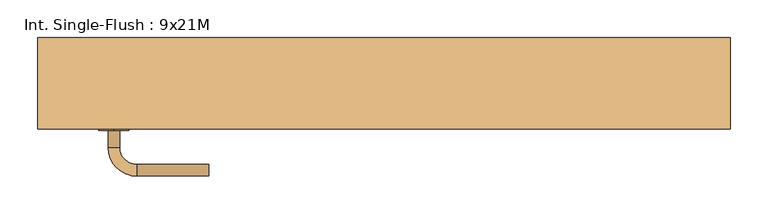
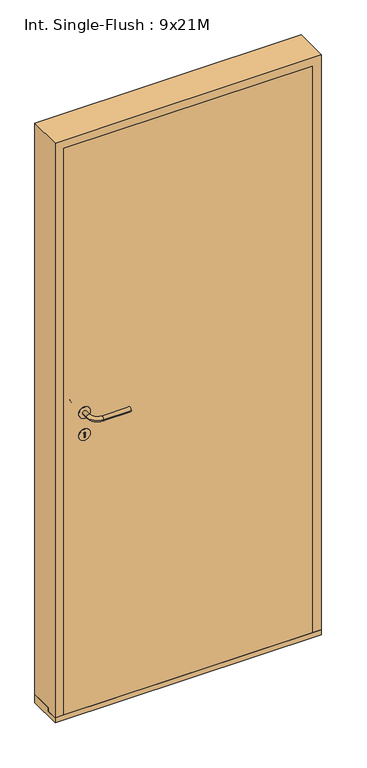
"""IFC4 building model written with IfcOpenShell, lengths in millimetres: door geometry, Int. Single-Flush : 9x21M."""

import ifcopenshell
import ifcopenshell.guid

model = None  # the IFC model being written
_history = None  # IfcOwnerHistory: only IFC2X3 demands one
_inside = {}  # id of a spatial element -> (the spatial element, [elements in it])
_under = {}  # id of a project, library or spatial element -> (it, [spatial elements below it])
_declared = {}  # id of a project -> (the project, [libraries it declares])
_typed = {}  # id of a type object -> (the type object, [elements of that type])
_made_of = {}  # id of a material, layer set ... -> (it, [elements and type objects made of it])


def new_model(schema):
    """Start an empty IFC model of exactly this schema.

    Asked for "IFC4X3", IfcOpenShell would pick the latest addendum, in which some entities
    have other attributes; the version numbers below select the first issue.
    IFC2X3 requires an IfcOwnerHistory on every rooted entity: one is made here for all.
    """
    global model, _history
    if schema == "IFC4X3":
        model = ifcopenshell.file(schema_version=(4, 3, 0, 0))
    else:
        model = ifcopenshell.file(schema=schema)
    _inside.clear()
    _under.clear()
    _declared.clear()
    _typed.clear()
    _made_of.clear()
    _history = None
    if model.schema == "IFC2X3":
        org = make("IfcOrganization", Name="unknown")
        user = make(
            "IfcPersonAndOrganization",
            ThePerson=make("IfcPerson", FamilyName="unknown"),
            TheOrganization=org,
        )
        app = make(
            "IfcApplication",
            ApplicationDeveloper=org,
            Version="unknown",
            ApplicationFullName="unknown",
            ApplicationIdentifier="unknown",
        )
        _history = make(
            "IfcOwnerHistory",
            OwningUser=user,
            OwningApplication=app,
            ChangeAction="ADDED",
            CreationDate=0,
        )
    return model


def make(cls, **values):
    """One entity of the class cls with the attributes given. An attribute that is None is left unset."""
    return model.create_entity(
        cls, **{name: value for name, value in values.items() if value is not None}
    )


def rooted(cls, **values):
    """An entity with a GlobalId (a new one), such as an element, a storey or a relation."""
    return make(cls, GlobalId=ifcopenshell.guid.new(), OwnerHistory=_history, **values)


def si_unit(unit_type, name, prefix=None):
    """IfcSIUnit, for example si_unit("LENGTHUNIT", "METRE", prefix="MILLI")."""
    return make("IfcSIUnit", UnitType=unit_type, Prefix=prefix, Name=name)


def assignment(units):
    """IfcUnitAssignment: the units of a project."""
    return None if units is None else make("IfcUnitAssignment", Units=units)


def point(xyz):
    """IfcCartesianPoint."""
    return None if xyz is None else make("IfcCartesianPoint", Coordinates=xyz)


def direction(xyz):
    """IfcDirection."""
    return None if xyz is None else make("IfcDirection", DirectionRatios=xyz)


def frame(location, z_axis=None, x_axis=None):
    """IfcAxis2Placement3D, a coordinate frame: its origin and axes. An axis left out is left unset."""
    return make(
        "IfcAxis2Placement3D",
        Location=point(location),
        Axis=direction(z_axis),
        RefDirection=direction(x_axis),
    )


def frame_2d(location, x_axis=None):
    """IfcAxis2Placement2D, a coordinate frame in the plane: its origin and x axis."""
    return make(
        "IfcAxis2Placement2D", Location=point(location), RefDirection=direction(x_axis)
    )


def origin():
    """The frame at (0, 0, 0) with its axes left unset."""
    return frame((0.0, 0.0, 0.0))


def place(relative_to, where):
    """IfcLocalPlacement: puts the frame where relative to a parent placement (None: the world)."""
    return make(
        "IfcLocalPlacement", PlacementRelTo=relative_to, RelativePlacement=where
    )


def context(
    kind, dimensions, precision=None, world=None, true_north=None, identifier=None
):
    """IfcGeometricRepresentationContext, for example the 3D "Model" context."""
    return make(
        "IfcGeometricRepresentationContext",
        ContextIdentifier=identifier,
        ContextType=kind,
        CoordinateSpaceDimension=dimensions,
        Precision=precision,
        WorldCoordinateSystem=world,
        TrueNorth=true_north,
    )


def project(units=None, contexts=None):
    """IfcProject with its units and contexts."""
    return rooted(
        "IfcProject",
        Name="project",
        RepresentationContexts=contexts,
        UnitsInContext=assignment(units),
    )


def spatial(cls, under=None, at=None, **own):
    """A site, building, storey or space (cls), placed at a placement, below another one or the project."""
    s = rooted(cls, ObjectPlacement=at, **own)
    if under is not None:
        _under.setdefault(under.id(), (under, []))[1].append(s)
    return s


def polyline(points):
    """IfcPolyline through the points."""
    return make("IfcPolyline", Points=[point(p) for p in points])


def circle_curve(where, radius):
    """IfcCircle in the frame where."""
    return make("IfcCircle", Position=where, Radius=radius)


def ellipse_curve(where, semi_axis1, semi_axis2):
    """IfcEllipse in the frame where."""
    return make(
        "IfcEllipse", Position=where, SemiAxis1=semi_axis1, SemiAxis2=semi_axis2
    )


def trimmed(basis, trim1, trim2, sense, master):
    """IfcTrimmedCurve: the piece of a basis curve between two trims."""
    return make(
        "IfcTrimmedCurve",
        BasisCurve=basis,
        Trim1=trim1,
        Trim2=trim2,
        SenseAgreement=sense,
        MasterRepresentation=master,
    )


def segment(curve, same_sense, transition):
    """IfcCompositeCurveSegment."""
    return make(
        "IfcCompositeCurveSegment",
        Transition=transition,
        SameSense=same_sense,
        ParentCurve=curve,
    )


def composite_curve(segments, self_intersect=None):
    """IfcCompositeCurve: segments joined end to end."""
    return make("IfcCompositeCurve", Segments=segments, SelfIntersect=self_intersect)


def outline(outer, holes=None, kind="AREA"):
    """IfcArbitraryClosedProfileDef: a profile drawn as a closed curve; with holes, ...WithVoids."""
    if holes is None:
        return make("IfcArbitraryClosedProfileDef", ProfileType=kind, OuterCurve=outer)
    return make(
        "IfcArbitraryProfileDefWithVoids",
        ProfileType=kind,
        OuterCurve=outer,
        InnerCurves=holes,
    )


def extrude(swept, where, along, depth):
    """IfcExtrudedAreaSolid: the profile swept, set in the frame where, extruded along a direction by depth."""
    return make(
        "IfcExtrudedAreaSolid",
        SweptArea=swept,
        Position=where,
        ExtrudedDirection=direction(along),
        Depth=depth,
    )


def faces_of(points, faces, orient=None, outer=None):
    """IfcFace entities. A face is a list of loops; a loop is a list of indices into points, from 0.

    orient and outer hold one flag for each loop. By default every Orientation is true, the
    first loop of a face is its IfcFaceOuterBound and the others are IfcFaceBound.
    """
    made = []
    for i, loops in enumerate(faces):
        bounds = []
        for j, loop in enumerate(loops):
            is_outer = j == 0 if outer is None else outer[i][j]
            bounds.append(
                make(
                    "IfcFaceOuterBound" if is_outer else "IfcFaceBound",
                    Bound=make("IfcPolyLoop", Polygon=[points[k] for k in loop]),
                    Orientation=True if orient is None else orient[i][j],
                )
            )
        made.append(make("IfcFace", Bounds=bounds))
    return made


def faceted_brep(points, faces, orient=None, outer=None, voids=None):
    """IfcFacetedBrep: a solid bounded by flat faces; with voids (closed shells), ...WithVoids."""
    shared = [point(p) for p in points]
    hull = make("IfcClosedShell", CfsFaces=faces_of(shared, faces, orient, outer))
    if voids is None:
        return make("IfcFacetedBrep", Outer=hull)
    return make(
        "IfcFacetedBrepWithVoids",
        Outer=hull,
        Voids=[
            make(cls, CfsFaces=faces_of(shared, fs, o, b)) for cls, fs, o, b in voids
        ],
    )


def shape(context_of_items, identifier, shape_type, items):
    """IfcShapeRepresentation: the items that make up one representation, for example the "Body"."""
    return make(
        "IfcShapeRepresentation",
        ContextOfItems=context_of_items,
        RepresentationIdentifier=identifier,
        RepresentationType=shape_type,
        Items=items,
    )


def source(mapping_origin, context_of_items, identifier, shape_type, items):
    """IfcRepresentationMap: a shape defined once, which mapped items show again and again."""
    return make(
        "IfcRepresentationMap",
        MappingOrigin=mapping_origin,
        MappedRepresentation=shape(context_of_items, identifier, shape_type, items),
    )


def transform(
    local_origin,
    x_axis=None,
    y_axis=None,
    z_axis=None,
    scale=None,
    scale2=None,
    scale3=None,
    uniform=True,
):
    """IfcCartesianTransformationOperator3D, or its non-uniform kind. x_axis, y_axis, z_axis: its Axis1, 2, 3."""
    if uniform:
        return make(
            "IfcCartesianTransformationOperator3D",
            Axis1=direction(x_axis),
            Axis2=direction(y_axis),
            LocalOrigin=point(local_origin),
            Scale=scale,
            Axis3=direction(z_axis),
        )
    return make(
        "IfcCartesianTransformationOperator3DnonUniform",
        Axis1=direction(x_axis),
        Axis2=direction(y_axis),
        LocalOrigin=point(local_origin),
        Scale=scale,
        Axis3=direction(z_axis),
        Scale2=scale2,
        Scale3=scale3,
    )


def mapped(mapping_source, mapping_target):
    """IfcMappedItem: shows the shape of a source again, moved by a transform."""
    return make(
        "IfcMappedItem", MappingSource=mapping_source, MappingTarget=mapping_target
    )


def made_of(thing, what):
    """Note that an element or type object is made of a material, layer set ...; save() writes the relation."""
    if what is not None:
        _made_of.setdefault(what.id(), (what, []))[1].append(thing)
    return thing


def element(
    cls,
    number,
    at=None,
    inside=None,
    cuts=None,
    type_object=None,
    material=None,
    context=None,
    identifier="Body",
    shape_type=None,
    held_by="IfcProductDefinitionShape",
    body=None,
    shapes=None,
    **own,
):
    """One element of the class cls, such as IfcWall. Its Tag is "e" and its number.

    at: its placement. inside: the storey or other place that contains it. cuts: it is an
    opening in that element (IfcRelVoidsElement). A single representation is given by context,
    identifier, shape_type and body (its items); several are given by shapes. held_by: the class
    of the entity that holds the representations. save() writes the other relations.
    """
    e = rooted(cls, Tag="e%d" % number, ObjectPlacement=at, **own)
    if body is not None:
        shapes = [shape(context, identifier, shape_type, body)]
    if shapes is not None:
        e.Representation = make(held_by, Representations=shapes)
    if inside is not None:
        _inside.setdefault(inside.id(), (inside, []))[1].append(e)
    if cuts is not None:
        rooted(
            "IfcRelVoidsElement", RelatingBuildingElement=cuts, RelatedOpeningElement=e
        )
    if type_object is not None:
        _typed.setdefault(type_object.id(), (type_object, []))[1].append(e)
    return made_of(e, material)


def aggregate(whole, parts):
    """IfcRelAggregates: a whole, such as a stair, and the parts it consists of."""
    return rooted("IfcRelAggregates", RelatingObject=whole, RelatedObjects=parts)


def save(model, path):
    """Write the relations noted so far, then the file.

    IfcRelAggregates (storeys below a building ...), IfcRelContainedInSpatialStructure (elements
    in a storey), IfcRelDefinesByType, IfcRelAssociatesMaterial and IfcRelDeclares: one each for
    every whole, place, type object, material and project.
    """
    for whole, parts in _under.values():
        aggregate(whole, parts)
    for where, things in _inside.values():
        rooted(
            "IfcRelContainedInSpatialStructure",
            RelatedElements=things,
            RelatingStructure=where,
        )
    for kind, things in _typed.values():
        rooted("IfcRelDefinesByType", RelatedObjects=things, RelatingType=kind)
    for what, things in _made_of.values():
        rooted("IfcRelAssociatesMaterial", RelatedObjects=things, RelatingMaterial=what)
    for by, libraries in _declared.values():
        rooted("IfcRelDeclares", RelatingContext=by, RelatedDefinitions=libraries)
    model.write(path)


def plane_surface(at):
    """IfcPlane: the flat surface through the origin of the frame at, square to its z axis."""
    return make("IfcPlane", Position=at)


def cylinder_surface(at, radius):
    """IfcCylindricalSurface: all points at the distance radius from the z axis of the frame at."""
    return make("IfcCylindricalSurface", Position=at, Radius=radius)


def revolved_surface(curve, axis_point, axis_direction):
    """IfcSurfaceOfRevolution: the curve turned about the line through axis_point along axis_direction."""
    return make(
        "IfcSurfaceOfRevolution",
        SweptCurve=make("IfcArbitraryOpenProfileDef", ProfileType="CURVE", Curve=curve),
        AxisPosition=make("IfcAxis1Placement", Location=point(axis_point), Axis=direction(axis_direction)),
    )


def advanced_brep(points, edges, surfaces, faces):
    """IfcAdvancedBrep: a solid bounded by faces that lie on surfaces and meet in shared edges.

    An edge is (start, end): straight between two places in points (the first is 0);
    or (start, end, curve); or (start, end, curve, False) where it runs against its curve.
    A face is (place in surfaces, loops), or (place, loops, False) where it looks against
    its surface's normal. A loop lists edges by number (the first is 1), with a minus sign
    where the edge is run from its end to its start. The first loop is the outer one.
    """
    corners = [point(p) for p in points]
    vertices = [make("IfcVertexPoint", VertexGeometry=c) for c in corners]
    made = []
    for start, end, *more in edges:
        made.append(
            make(
                "IfcEdgeCurve",
                EdgeStart=vertices[start],
                EdgeEnd=vertices[end],
                EdgeGeometry=more[0] if more else make("IfcPolyline", Points=[corners[start], corners[end]]),
                SameSense=more[1] if len(more) > 1 else True,
            )
        )
    hull = []
    for where, loops, *sense in faces:
        bounds = []
        for j, loop in enumerate(loops):
            ring = [make("IfcOrientedEdge", EdgeElement=made[abs(k) - 1], Orientation=k > 0) for k in loop]
            bounds.append(
                make(
                    "IfcFaceOuterBound" if j == 0 else "IfcFaceBound",
                    Bound=make("IfcEdgeLoop", EdgeList=ring),
                    Orientation=True,
                )
            )
        hull.append(make("IfcAdvancedFace", Bounds=bounds, FaceSurface=surfaces[where], SameSense=sense[0] if sense else True))
    return make("IfcAdvancedBrep", Outer=make("IfcClosedShell", CfsFaces=hull))


def int_single_flush_9x21m_9bb4a9f8(model_context):
    return source(origin(), model_context, "Body", "SolidModel", [
        extrude(outline(composite_curve([segment(trimmed(circle_curve(frame_2d((1090.0, -356.0)), 20.0), [point((1070.0, -356.0))], [point((1110.0, -356.0))], False, "CARTESIAN"), True, "CONTINUOUS"), segment(trimmed(circle_curve(frame_2d((1090.0, -356.0)), 20.0), [point((1110.0, -356.0))], [point((1070.0, -356.0))], False, "CARTESIAN"), True, "CONTINUOUS")], self_intersect=False)), frame((0.0, -62.0, 0.0), z_axis=(0.0, 1.0, 0.0), x_axis=(0.0, 0.0, 1.0)), (0.0, 0.0, 1.0), 2.0),
        advanced_brep(
        [(-363.5, -62.0, 1090.0), (-348.5, -62.0, 1090.0), (-348.5, -84.5, 1090.0), (-363.5, -84.5, 1090.0), (-326.0, -107.0, 1090.0), (-326.0, -122.0, 1090.0), (-231.0, -107.0, 1090.0), (-231.0, -122.0, 1090.0)],
        [
            (0, 1, circle_curve(frame((-356.0, -62.0, 1090.0), z_axis=(0.0, 1.0, 0.0), x_axis=(1.0, 0.0, 0.0)), 7.5)),
            (1, 0, circle_curve(frame((-356.0, -62.0, 1090.0), z_axis=(0.0, 1.0, 0.0), x_axis=(1.0, 0.0, 0.0)), 7.5)),
            (1, 2),
            (2, 3, circle_curve(frame((-356.0, -84.5, 1090.0), z_axis=(0.0, 1.0, 0.0), x_axis=(1.0, 0.0, 0.0)), 7.5)),
            (3, 0),
            (3, 2, circle_curve(frame((-356.0, -84.5, 1090.0), z_axis=(0.0, 1.0, 0.0), x_axis=(1.0, 0.0, 0.0)), 7.5)),
            (4, 5, circle_curve(frame((-326.0, -114.5, 1090.0), z_axis=(-1.0, 0.0, 0.0), x_axis=(0.0, 1.0, 0.0)), 7.5)),
            (5, 3, circle_curve(frame((-326.0, -84.5, 1090.0), z_axis=(0.0, 0.0, -1.0), x_axis=(-1.0, 0.0, 0.0)), 37.5)),
            (2, 4, circle_curve(frame((-326.0, -84.5, 1090.0), z_axis=(0.0, 0.0, 1.0), x_axis=(-1.0, 0.0, 0.0)), 22.5)),
            (5, 4, circle_curve(frame((-326.0, -114.5, 1090.0), z_axis=(-1.0, 0.0, 0.0), x_axis=(0.0, 1.0, 0.0)), 7.5)),
            (4, 6),
            (6, 7, circle_curve(frame((-231.0, -114.5, 1090.0), z_axis=(-1.0, 0.0, 0.0), x_axis=(0.0, 1.0, 0.0)), 7.5)),
            (7, 5),
            (7, 6, circle_curve(frame((-231.0, -114.5, 1090.0), z_axis=(-1.0, 0.0, 0.0), x_axis=(0.0, 1.0, 0.0)), 7.5)),
        ],
        [
            plane_surface(frame((-356.0, -62.0, 1090.0), z_axis=(0.0, 1.0, 0.0), x_axis=(0.0, 0.0, -1.0))),
            cylinder_surface(frame((-356.0, -62.0, 1090.0), z_axis=(0.0, 1.0, 0.0), x_axis=(1.0, 0.0, 0.0)), 7.5),
            revolved_surface(trimmed(ellipse_curve(frame((-356.0, -84.5, 1090.0), z_axis=(0.0, -1.0, 0.0), x_axis=(1.0, 0.0, 0.0)), 7.5, 7.5), [point((-363.5, -84.5, 1090.0))], [point((-348.5, -84.5, 1090.0))], True, "CARTESIAN"), (-326.0, -84.5, 1090.0), (0.0, 0.0, -1.0)),
            revolved_surface(trimmed(ellipse_curve(frame((-356.0, -84.5, 1090.0), z_axis=(0.0, -1.0, 0.0), x_axis=(1.0, 0.0, 0.0)), 7.5, 7.5), [point((-348.5, -84.5, 1090.0))], [point((-363.5, -84.5, 1090.0))], True, "CARTESIAN"), (-326.0, -84.5, 1090.0), (0.0, 0.0, -1.0)),
            cylinder_surface(frame((-326.0, -114.5, 1090.0), z_axis=(-1.0, 0.0, 0.0), x_axis=(0.0, 1.0, 0.0)), 7.5),
            plane_surface(frame((-231.0, -114.5, 1090.0), z_axis=(1.0, 0.0, 0.0), x_axis=(0.0, 0.0, -1.0))),
        ],
        [
            (0, [[1, 2]]),
            (1, [[3, 4, 5, -2]]),
            (1, [[-5, 6, -3, -1]]),
            (2, [[7, 8, -4, 9]]),
            (3, [[10, -9, -6, -8]]),
            (4, [[11, 12, 13, -7]]),
            (4, [[-13, 14, -11, -10]]),
            (5, [[-12, -14]]),
        ],
    ),
        extrude(outline(composite_curve([segment(trimmed(circle_curve(frame_2d((1010.0, -356.0)), 20.0), [point((990.0, -356.0))], [point((1030.0, -356.0))], False, "CARTESIAN"), True, "CONTINUOUS"), segment(trimmed(circle_curve(frame_2d((1010.0, -356.0)), 20.0), [point((1030.0, -356.0))], [point((990.0, -356.0))], False, "CARTESIAN"), True, "CONTINUOUS")], self_intersect=False), holes=[composite_curve([segment(trimmed(circle_curve(frame_2d((1015.0, -356.0)), 3.0), [point((1012.4019238, -357.5))], [point((1012.4019238, -354.5))], True, "CARTESIAN"), True, "CONTINUOUS"), segment(polyline([(1012.4019238, -354.5), (1000.0, -354.5), (1000.0, -357.5), (1012.4019238, -357.5)]), True, "CONTINUOUS")], self_intersect=False)]), frame((0.0, -62.0, 0.0), z_axis=(0.0, 1.0, 0.0), x_axis=(0.0, 0.0, 1.0)), (0.0, 0.0, 1.0), 2.0),
        extrude(outline(composite_curve([segment(trimmed(circle_curve(frame_2d((1090.0, -356.0)), 20.0), [point((1070.0, -356.0))], [point((1110.0, -356.0))], False, "CARTESIAN"), True, "CONTINUOUS"), segment(trimmed(circle_curve(frame_2d((1090.0, -356.0)), 20.0), [point((1110.0, -356.0))], [point((1070.0, -356.0))], False, "CARTESIAN"), True, "CONTINUOUS")], self_intersect=False)), frame((0.0, -20.0, 0.0), z_axis=(0.0, 1.0, 0.0), x_axis=(0.0, 0.0, 1.0)), (0.0, 0.0, 1.0), 2.0),
        advanced_brep(
        [(-363.5, -18.0, 1090.0), (-348.5, -18.0, 1090.0), (-363.5, 4.5, 1090.0), (-348.5, 4.5, 1090.0), (-326.0, 27.0, 1090.0), (-326.0, 42.0, 1090.0), (-231.0, 42.0, 1090.0), (-231.0, 27.0, 1090.0)],
        [
            (0, 1, circle_curve(frame((-356.0, -18.0, 1090.0), z_axis=(0.0, -1.0, 0.0), x_axis=(1.0, 0.0, 0.0)), 7.5)),
            (1, 0, circle_curve(frame((-356.0, -18.0, 1090.0), z_axis=(0.0, -1.0, 0.0), x_axis=(1.0, 0.0, 0.0)), 7.5)),
            (0, 2),
            (2, 3, circle_curve(frame((-356.0, 4.5, 1090.0), z_axis=(0.0, -1.0, 0.0), x_axis=(1.0, 0.0, 0.0)), 7.5)),
            (3, 1),
            (3, 2, circle_curve(frame((-356.0, 4.5, 1090.0), z_axis=(0.0, -1.0, 0.0), x_axis=(1.0, 0.0, 0.0)), 7.5)),
            (4, 3, circle_curve(frame((-326.0, 4.5, 1090.0), z_axis=(0.0, 0.0, 1.0), x_axis=(-1.0, 0.0, 0.0)), 22.5)),
            (2, 5, circle_curve(frame((-326.0, 4.5, 1090.0), z_axis=(0.0, 0.0, -1.0), x_axis=(-1.0, 0.0, 0.0)), 37.5)),
            (5, 4, circle_curve(frame((-326.0, 34.5, 1090.0), z_axis=(-1.0, 0.0, 0.0), x_axis=(0.0, -1.0, 0.0)), 7.5)),
            (4, 5, circle_curve(frame((-326.0, 34.5, 1090.0), z_axis=(-1.0, 0.0, 0.0), x_axis=(0.0, -1.0, 0.0)), 7.5)),
            (5, 6),
            (6, 7, circle_curve(frame((-231.0, 34.5, 1090.0), z_axis=(-1.0, 0.0, 0.0), x_axis=(0.0, -1.0, 0.0)), 7.5)),
            (7, 4),
            (7, 6, circle_curve(frame((-231.0, 34.5, 1090.0), z_axis=(-1.0, 0.0, 0.0), x_axis=(0.0, -1.0, 0.0)), 7.5)),
        ],
        [
            plane_surface(frame((-356.0, -18.0, 1090.0), z_axis=(0.0, -1.0, 0.0), x_axis=(0.0, 0.0, -1.0))),
            cylinder_surface(frame((-356.0, -18.0, 1090.0), z_axis=(0.0, -1.0, 0.0), x_axis=(1.0, 0.0, 0.0)), 7.5),
            revolved_surface(trimmed(ellipse_curve(frame((-356.0, 4.5, 1090.0), z_axis=(0.0, -1.0, 0.0), x_axis=(1.0, 0.0, 0.0)), 7.5, 7.5), [point((-363.5, 4.5, 1090.0))], [point((-348.5, 4.5, 1090.0))], True, "CARTESIAN"), (-326.0, 4.5, 1090.0), (0.0, 0.0, -1.0)),
            revolved_surface(trimmed(ellipse_curve(frame((-356.0, 4.5, 1090.0), z_axis=(0.0, -1.0, 0.0), x_axis=(1.0, 0.0, 0.0)), 7.5, 7.5), [point((-348.5, 4.5, 1090.0))], [point((-363.5, 4.5, 1090.0))], True, "CARTESIAN"), (-326.0, 4.5, 1090.0), (0.0, 0.0, -1.0)),
            cylinder_surface(frame((-326.0, 34.5, 1090.0), z_axis=(-1.0, 0.0, 0.0), x_axis=(0.0, -1.0, 0.0)), 7.5),
            plane_surface(frame((-231.0, 34.5, 1090.0), z_axis=(1.0, 0.0, 0.0), x_axis=(0.0, 0.0, -1.0))),
        ],
        [
            (0, [[1, 2]]),
            (1, [[-1, 3, 4, 5]]),
            (1, [[-2, -5, 6, -3]]),
            (2, [[7, -4, 8, 9]]),
            (3, [[-8, -6, -7, 10]]),
            (4, [[-9, 11, 12, 13]]),
            (4, [[-10, -13, 14, -11]]),
            (5, [[-14, -12]]),
        ],
    ),
        extrude(outline(composite_curve([segment(trimmed(circle_curve(frame_2d((1010.0, -356.0)), 20.0), [point((990.0, -356.0))], [point((1030.0, -356.0))], False, "CARTESIAN"), True, "CONTINUOUS"), segment(trimmed(circle_curve(frame_2d((1010.0, -356.0)), 20.0), [point((1030.0, -356.0))], [point((990.0, -356.0))], False, "CARTESIAN"), True, "CONTINUOUS")], self_intersect=False), holes=[composite_curve([segment(trimmed(circle_curve(frame_2d((1015.0, -356.0)), 3.0), [point((1012.4019238, -357.5))], [point((1012.4019238, -354.5))], True, "CARTESIAN"), True, "CONTINUOUS"), segment(polyline([(1012.4019238, -354.5), (1000.0, -354.5), (1000.0, -357.5), (1012.4019238, -357.5)]), True, "CONTINUOUS")], self_intersect=False)]), frame((0.0, -20.0, 0.0), z_axis=(0.0, 1.0, 0.0), x_axis=(0.0, 0.0, 1.0)), (0.0, 0.0, 1.0), 2.0),
        extrude(outline(polyline([(426.0, -20.0), (426.0, -60.0), (-426.0, -60.0), (-426.0, -20.0), (426.0, -20.0)])), frame((0.0, 0.0, 18.0), z_axis=(0.0, 0.0, 1.0), x_axis=(1.0, 0.0, 0.0)), (0.0, 0.0, 1.0), 2052.0),
        faceted_brep([(-426.0, -20.0, 2070.0), (-426.0, -20.0, 30.0), (-414.0, -20.0, 30.0), (-414.0, -20.0, 2058.0), (414.0, -20.0, 2058.0), (414.0, -20.0, 30.0), (426.0, -20.0, 30.0), (426.0, -20.0, 2070.0), (-426.0, -60.0, 2070.0), (-426.0, -60.0, 18.0), (-426.0, -20.0, 18.0), (-456.0, -20.0, 18.0), (-456.0, -20.0, 30.0), (456.0, -20.0, 30.0), (456.0, -20.0, 18.0), (426.0, -20.0, 18.0), (-456.0, -60.0, 18.0), (456.0, -60.0, 18.0), (426.0, -60.0, 18.0), (-456.0, -60.0, 2100.0), (426.0, -60.0, 2070.0), (456.0, -60.0, 2100.0), (414.0, 60.0, 30.0), (456.0, 60.0, 30.0), (-456.0, 60.0, 30.0), (-414.0, 60.0, 30.0), (414.0, 60.0, 2058.0), (-414.0, 60.0, 2058.0), (-456.0, 60.0, 2100.0), (456.0, 60.0, 2100.0)], [[[0, 1, 2, 3, 4, 5, 6, 7]], [[8, 9, 10, 1, 0]], [[1, 10, 11, 12]], [[13, 14, 15, 6]], [[10, 9, 16, 11]], [[14, 17, 18, 15]], [[19, 16, 9, 8, 20, 18, 17, 21]], [[7, 6, 15, 18, 20]], [[6, 5, 22, 23, 13]], [[12, 24, 25, 2, 1]], [[26, 22, 5, 4]], [[3, 2, 25, 27]], [[27, 25, 24, 28, 29, 23, 22, 26]], [[21, 17, 14, 13, 23, 29]], [[28, 24, 12, 11, 16, 19]], [[0, 7, 20, 8]], [[3, 27, 26, 4]], [[28, 19, 21, 29]]]),
        extrude(outline(polyline([(-20.0, 30.0), (60.0, 30.0), (60.0, 0.0), (-60.0, 0.0), (-60.0, 18.0), (-20.0, 18.0), (-20.0, 30.0)])), frame((-456.0, 0.0, 0.0), z_axis=(1.0, 0.0, 0.0), x_axis=(0.0, 1.0, 0.0)), (0.0, 0.0, 1.0), 912.0),
    ])


if __name__ == "__main__":
    model = new_model("IFC4")
    model_context = context("Model", 3, world=origin())
    ifc_project = project(units=[si_unit("LENGTHUNIT", "METRE", prefix="MILLI")], contexts=[model_context])
    site = spatial("IfcSite", under=ifc_project)
    building = spatial("IfcBuilding", under=site)
    placement = place(None, origin())
    int_single_flush_9x21m_shape = int_single_flush_9x21m_9bb4a9f8(model_context)
    element("IfcDoor", 1, ObjectType="Int. Single-Flush : 9x21M", at=placement, inside=building, context=model_context, shape_type="MappedRepresentation", body=[
        mapped(int_single_flush_9x21m_shape, transform((0.0, 0.0, 0.0), x_axis=(1.0, 0.0, 0.0), y_axis=(0.0, 1.0, 0.0), z_axis=(0.0, 0.0, 1.0))),
    ])
    save(model, "model.ifc")

# Revit data of these elements
# Type "Int. Single-Flush : 9x21M"
#   Type Mark = "53"
#   Sound Rating = ""
#   Hinge Side [instance default] = ""
#   Creator Build [instance default] = "2017.0301.0"
#   Creator Organization [instance default] = "© Danish Educational Content"
#   Creator Name [instance default] = "© Erik Falck Jørgensen"
#   Analytic Construction = "<None>"
#   length#3 = 18 mm
#   length#2 = 42 mm
#   length#1 = 0 mm
#   length#4 = 912 mm
#   Thickness = 40 mm
#   Seal Width = 12 mm
#   Rough Width = 912 mm
#   Rough Height = 2100 mm
#   Rabbet Width = 12 mm
#   Rabbet Depth = 40 mm
#   Interior Distance [instance default] = 0 mm
#   Height = 2088 mm
#   Width = 888 mm
#   Handle From Side = 100 mm
#   Handle From Bottom = 1090 mm
#   Exterior Direction [instance default] = 0.00°
#   Case Depth [instance default] = 200 mm
#   Case Width = 30 mm
#   Exterior Distance [instance default] = 0 mm
#   Threshold = yes
#   Sealing = no
#   Hinging = yes
#   Wall Closure = 1
#   Door Panel = no
#   Panel = none
#   Handle Finish = none
#   Handle = element 510752
#   Case/Transom = none
#   Function = (empty or 0)
#   Assembly Code = ""
# Element 1 (IfcDoor, "Int. Single-Flush : 9x21M")
#   Case Depth = 120 mm
#   Materials on its faces: "Stainless Steel, Polished", "Default Frame/Mullion (Interior/Exterior)", "Default Door Panel (Exterior/Interior)"
# Materials
#   "Stainless Steel, Polished": class "Metal", colour RGB 180 180 180, transparency 0, Description = "Rustfri stål, poleret", Cost = 0
#   "Default Frame/Mullion (Interior/Exterior)": class "Generic", colour RGB 205 205 205, transparency 0, Description = "Udefineret karm/ramme materiale", Cost = 0
#   "Default Door Panel (Exterior/Interior)": class "Generic", colour RGB 205 205 205, transparency 0, Description = "Udefineret dørplade materiale", Cost = 0
